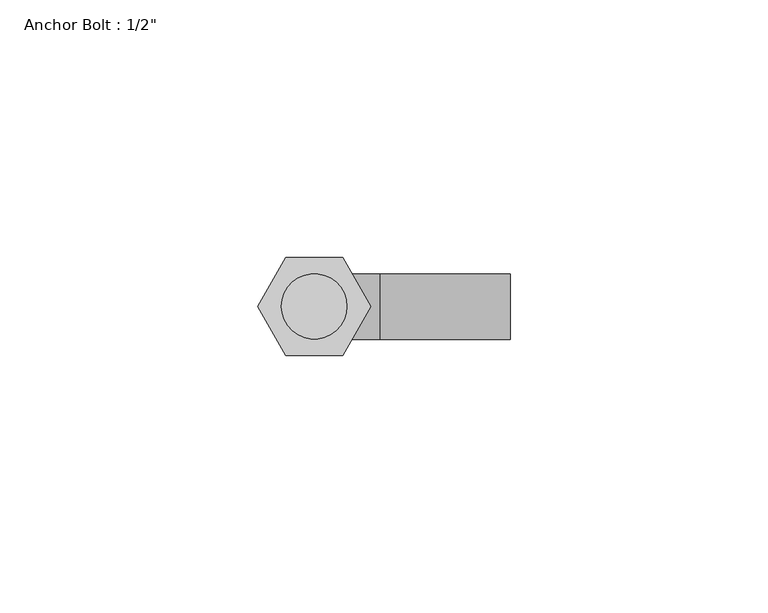
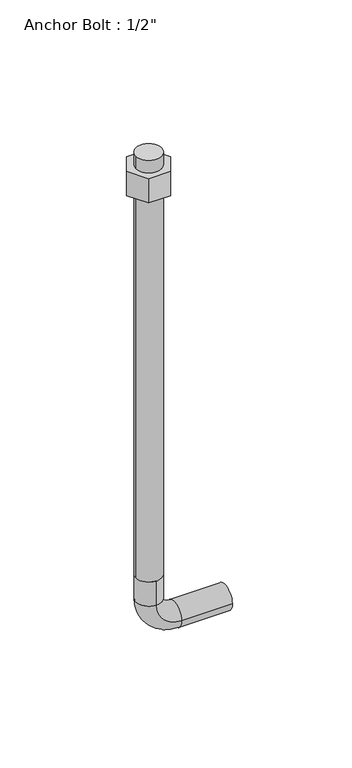
"""IFC4 building model written with IfcOpenShell, lengths in millimetres: fastener geometry."""

import ifcopenshell
import ifcopenshell.guid

model = None  # the IFC model being written
_history = None  # IfcOwnerHistory: only IFC2X3 demands one
_inside = {}  # id of a spatial element -> (the spatial element, [elements in it])
_under = {}  # id of a project, library or spatial element -> (it, [spatial elements below it])
_declared = {}  # id of a project -> (the project, [libraries it declares])
_typed = {}  # id of a type object -> (the type object, [elements of that type])
_made_of = {}  # id of a material, layer set ... -> (it, [elements and type objects made of it])


def new_model(schema):
    """Start an empty IFC model of exactly this schema.

    Asked for "IFC4X3", IfcOpenShell would pick the latest addendum, in which some entities
    have other attributes; the version numbers below select the first issue.
    IFC2X3 requires an IfcOwnerHistory on every rooted entity: one is made here for all.
    """
    global model, _history
    if schema == "IFC4X3":
        model = ifcopenshell.file(schema_version=(4, 3, 0, 0))
    else:
        model = ifcopenshell.file(schema=schema)
    _inside.clear()
    _under.clear()
    _declared.clear()
    _typed.clear()
    _made_of.clear()
    _history = None
    if model.schema == "IFC2X3":
        org = make("IfcOrganization", Name="unknown")
        user = make(
            "IfcPersonAndOrganization",
            ThePerson=make("IfcPerson", FamilyName="unknown"),
            TheOrganization=org,
        )
        app = make(
            "IfcApplication",
            ApplicationDeveloper=org,
            Version="unknown",
            ApplicationFullName="unknown",
            ApplicationIdentifier="unknown",
        )
        _history = make(
            "IfcOwnerHistory",
            OwningUser=user,
            OwningApplication=app,
            ChangeAction="ADDED",
            CreationDate=0,
        )
    return model


def make(cls, **values):
    """One entity of the class cls with the attributes given. An attribute that is None is left unset."""
    return model.create_entity(
        cls, **{name: value for name, value in values.items() if value is not None}
    )


def rooted(cls, **values):
    """An entity with a GlobalId (a new one), such as an element, a storey or a relation."""
    return make(cls, GlobalId=ifcopenshell.guid.new(), OwnerHistory=_history, **values)


def si_unit(unit_type, name, prefix=None):
    """IfcSIUnit, for example si_unit("LENGTHUNIT", "METRE", prefix="MILLI")."""
    return make("IfcSIUnit", UnitType=unit_type, Prefix=prefix, Name=name)


def assignment(units):
    """IfcUnitAssignment: the units of a project."""
    return None if units is None else make("IfcUnitAssignment", Units=units)


def point(xyz):
    """IfcCartesianPoint."""
    return None if xyz is None else make("IfcCartesianPoint", Coordinates=xyz)


def direction(xyz):
    """IfcDirection."""
    return None if xyz is None else make("IfcDirection", DirectionRatios=xyz)


def frame(location, z_axis=None, x_axis=None):
    """IfcAxis2Placement3D, a coordinate frame: its origin and axes. An axis left out is left unset."""
    return make(
        "IfcAxis2Placement3D",
        Location=point(location),
        Axis=direction(z_axis),
        RefDirection=direction(x_axis),
    )


def origin():
    """The frame at (0, 0, 0) with its axes left unset."""
    return frame((0.0, 0.0, 0.0))


def origin_with_axes():
    """The frame at (0, 0, 0) with the z axis (0, 0, 1) and the x axis (1, 0, 0) written out."""
    return frame((0.0, 0.0, 0.0), z_axis=(0.0, 0.0, 1.0), x_axis=(1.0, 0.0, 0.0))


def place(relative_to, where):
    """IfcLocalPlacement: puts the frame where relative to a parent placement (None: the world)."""
    return make(
        "IfcLocalPlacement", PlacementRelTo=relative_to, RelativePlacement=where
    )


def context(
    kind, dimensions, precision=None, world=None, true_north=None, identifier=None
):
    """IfcGeometricRepresentationContext, for example the 3D "Model" context."""
    return make(
        "IfcGeometricRepresentationContext",
        ContextIdentifier=identifier,
        ContextType=kind,
        CoordinateSpaceDimension=dimensions,
        Precision=precision,
        WorldCoordinateSystem=world,
        TrueNorth=true_north,
    )


def project(units=None, contexts=None):
    """IfcProject with its units and contexts."""
    return rooted(
        "IfcProject",
        Name="project",
        RepresentationContexts=contexts,
        UnitsInContext=assignment(units),
    )


def spatial(cls, under=None, at=None, **own):
    """A site, building, storey or space (cls), placed at a placement, below another one or the project."""
    s = rooted(cls, ObjectPlacement=at, **own)
    if under is not None:
        _under.setdefault(under.id(), (under, []))[1].append(s)
    return s


def polyline(points):
    """IfcPolyline through the points."""
    return make("IfcPolyline", Points=[point(p) for p in points])


def circle_curve(where, radius):
    """IfcCircle in the frame where."""
    return make("IfcCircle", Position=where, Radius=radius)


def ellipse_curve(where, semi_axis1, semi_axis2):
    """IfcEllipse in the frame where."""
    return make(
        "IfcEllipse", Position=where, SemiAxis1=semi_axis1, SemiAxis2=semi_axis2
    )


def trimmed(basis, trim1, trim2, sense, master):
    """IfcTrimmedCurve: the piece of a basis curve between two trims."""
    return make(
        "IfcTrimmedCurve",
        BasisCurve=basis,
        Trim1=trim1,
        Trim2=trim2,
        SenseAgreement=sense,
        MasterRepresentation=master,
    )


def outline(outer, holes=None, kind="AREA"):
    """IfcArbitraryClosedProfileDef: a profile drawn as a closed curve; with holes, ...WithVoids."""
    if holes is None:
        return make("IfcArbitraryClosedProfileDef", ProfileType=kind, OuterCurve=outer)
    return make(
        "IfcArbitraryProfileDefWithVoids",
        ProfileType=kind,
        OuterCurve=outer,
        InnerCurves=holes,
    )


def extrude(swept, where, along, depth):
    """IfcExtrudedAreaSolid: the profile swept, set in the frame where, extruded along a direction by depth."""
    return make(
        "IfcExtrudedAreaSolid",
        SweptArea=swept,
        Position=where,
        ExtrudedDirection=direction(along),
        Depth=depth,
    )


def shape(context_of_items, identifier, shape_type, items):
    """IfcShapeRepresentation: the items that make up one representation, for example the "Body"."""
    return make(
        "IfcShapeRepresentation",
        ContextOfItems=context_of_items,
        RepresentationIdentifier=identifier,
        RepresentationType=shape_type,
        Items=items,
    )


def source(mapping_origin, context_of_items, identifier, shape_type, items):
    """IfcRepresentationMap: a shape defined once, which mapped items show again and again."""
    return make(
        "IfcRepresentationMap",
        MappingOrigin=mapping_origin,
        MappedRepresentation=shape(context_of_items, identifier, shape_type, items),
    )


def transform(
    local_origin,
    x_axis=None,
    y_axis=None,
    z_axis=None,
    scale=None,
    scale2=None,
    scale3=None,
    uniform=True,
):
    """IfcCartesianTransformationOperator3D, or its non-uniform kind. x_axis, y_axis, z_axis: its Axis1, 2, 3."""
    if uniform:
        return make(
            "IfcCartesianTransformationOperator3D",
            Axis1=direction(x_axis),
            Axis2=direction(y_axis),
            LocalOrigin=point(local_origin),
            Scale=scale,
            Axis3=direction(z_axis),
        )
    return make(
        "IfcCartesianTransformationOperator3DnonUniform",
        Axis1=direction(x_axis),
        Axis2=direction(y_axis),
        LocalOrigin=point(local_origin),
        Scale=scale,
        Axis3=direction(z_axis),
        Scale2=scale2,
        Scale3=scale3,
    )


def mapped(mapping_source, mapping_target):
    """IfcMappedItem: shows the shape of a source again, moved by a transform."""
    return make(
        "IfcMappedItem", MappingSource=mapping_source, MappingTarget=mapping_target
    )


def made_of(thing, what):
    """Note that an element or type object is made of a material, layer set ...; save() writes the relation."""
    if what is not None:
        _made_of.setdefault(what.id(), (what, []))[1].append(thing)
    return thing


def element(
    cls,
    number,
    at=None,
    inside=None,
    cuts=None,
    type_object=None,
    material=None,
    context=None,
    identifier="Body",
    shape_type=None,
    held_by="IfcProductDefinitionShape",
    body=None,
    shapes=None,
    **own,
):
    """One element of the class cls, such as IfcWall. Its Tag is "e" and its number.

    at: its placement. inside: the storey or other place that contains it. cuts: it is an
    opening in that element (IfcRelVoidsElement). A single representation is given by context,
    identifier, shape_type and body (its items); several are given by shapes. held_by: the class
    of the entity that holds the representations. save() writes the other relations.
    """
    e = rooted(cls, Tag="e%d" % number, ObjectPlacement=at, **own)
    if body is not None:
        shapes = [shape(context, identifier, shape_type, body)]
    if shapes is not None:
        e.Representation = make(held_by, Representations=shapes)
    if inside is not None:
        _inside.setdefault(inside.id(), (inside, []))[1].append(e)
    if cuts is not None:
        rooted(
            "IfcRelVoidsElement", RelatingBuildingElement=cuts, RelatedOpeningElement=e
        )
    if type_object is not None:
        _typed.setdefault(type_object.id(), (type_object, []))[1].append(e)
    return made_of(e, material)


def aggregate(whole, parts):
    """IfcRelAggregates: a whole, such as a stair, and the parts it consists of."""
    return rooted("IfcRelAggregates", RelatingObject=whole, RelatedObjects=parts)


def save(model, path):
    """Write the relations noted so far, then the file.

    IfcRelAggregates (storeys below a building ...), IfcRelContainedInSpatialStructure (elements
    in a storey), IfcRelDefinesByType, IfcRelAssociatesMaterial and IfcRelDeclares: one each for
    every whole, place, type object, material and project.
    """
    for whole, parts in _under.values():
        aggregate(whole, parts)
    for where, things in _inside.values():
        rooted(
            "IfcRelContainedInSpatialStructure",
            RelatedElements=things,
            RelatingStructure=where,
        )
    for kind, things in _typed.values():
        rooted("IfcRelDefinesByType", RelatedObjects=things, RelatingType=kind)
    for what, things in _made_of.values():
        rooted("IfcRelAssociatesMaterial", RelatedObjects=things, RelatingMaterial=what)
    for by, libraries in _declared.values():
        rooted("IfcRelDeclares", RelatingContext=by, RelatedDefinitions=libraries)
    model.write(path)


def plane_surface(at):
    """IfcPlane: the flat surface through the origin of the frame at, square to its z axis."""
    return make("IfcPlane", Position=at)


def cylinder_surface(at, radius):
    """IfcCylindricalSurface: all points at the distance radius from the z axis of the frame at."""
    return make("IfcCylindricalSurface", Position=at, Radius=radius)


def revolved_surface(curve, axis_point, axis_direction):
    """IfcSurfaceOfRevolution: the curve turned about the line through axis_point along axis_direction."""
    return make(
        "IfcSurfaceOfRevolution",
        SweptCurve=make("IfcArbitraryOpenProfileDef", ProfileType="CURVE", Curve=curve),
        AxisPosition=make("IfcAxis1Placement", Location=point(axis_point), Axis=direction(axis_direction)),
    )


def advanced_brep(points, edges, surfaces, faces):
    """IfcAdvancedBrep: a solid bounded by faces that lie on surfaces and meet in shared edges.

    An edge is (start, end): straight between two places in points (the first is 0);
    or (start, end, curve); or (start, end, curve, False) where it runs against its curve.
    A face is (place in surfaces, loops), or (place, loops, False) where it looks against
    its surface's normal. A loop lists edges by number (the first is 1), with a minus sign
    where the edge is run from its end to its start. The first loop is the outer one.
    """
    corners = [point(p) for p in points]
    vertices = [make("IfcVertexPoint", VertexGeometry=c) for c in corners]
    made = []
    for start, end, *more in edges:
        made.append(
            make(
                "IfcEdgeCurve",
                EdgeStart=vertices[start],
                EdgeEnd=vertices[end],
                EdgeGeometry=more[0] if more else make("IfcPolyline", Points=[corners[start], corners[end]]),
                SameSense=more[1] if len(more) > 1 else True,
            )
        )
    hull = []
    for where, loops, *sense in faces:
        bounds = []
        for j, loop in enumerate(loops):
            ring = [make("IfcOrientedEdge", EdgeElement=made[abs(k) - 1], Orientation=k > 0) for k in loop]
            bounds.append(
                make(
                    "IfcFaceOuterBound" if j == 0 else "IfcFaceBound",
                    Bound=make("IfcEdgeLoop", EdgeList=ring),
                    Orientation=True,
                )
            )
        hull.append(make("IfcAdvancedFace", Bounds=bounds, FaceSurface=surfaces[where], SameSense=sense[0] if sense else True))
    return make("IfcAdvancedBrep", Outer=make("IfcClosedShell", CfsFaces=hull))


def fastener_5f8ddbac(model_context):
    return source(origin(), model_context, "Body", "SolidModel", [
        advanced_brep(
        [(-6.35, 0.0, 19.05), (6.35, 0.0, 19.05), (-6.35, 0.0, -203.2), (0.0, -6.35, -203.2), (6.35, 0.0, -203.2), (0.0, 6.35, -203.2), (0.0, 6.35, -215.9), (0.0, -6.35, -215.9), (12.7, 6.35, -228.6), (12.7, -6.35, -228.6), (38.1, 6.35, -228.6), (38.1, -6.35, -228.6)],
        [
            (0, 1, circle_curve(frame((0.0, 0.0, 19.05), z_axis=(0.0, 0.0, 1.0), x_axis=(1.0, 0.0, 0.0)), 6.35)),
            (1, 0, circle_curve(frame((0.0, 0.0, 19.05), z_axis=(0.0, 0.0, 1.0), x_axis=(1.0, 0.0, 0.0)), 6.35)),
            (0, 2),
            (2, 3, circle_curve(frame((0.0, 0.0, -203.2), z_axis=(0.0, 0.0, 1.0), x_axis=(1.0, 0.0, 0.0)), 6.35)),
            (3, 4, circle_curve(frame((0.0, 0.0, -203.2), z_axis=(0.0, 0.0, 1.0), x_axis=(1.0, 0.0, 0.0)), 6.35)),
            (4, 1),
            (4, 5, circle_curve(frame((0.0, 0.0, -203.2), z_axis=(0.0, 0.0, 1.0), x_axis=(1.0, 0.0, 0.0)), 6.35)),
            (5, 2, circle_curve(frame((0.0, 0.0, -203.2), z_axis=(0.0, 0.0, 1.0), x_axis=(1.0, 0.0, 0.0)), 6.35)),
            (5, 6),
            (6, 7, circle_curve(frame((0.0, 0.0, -215.9), z_axis=(0.0, 0.0, 1.0), x_axis=(0.0, -1.0, 0.0)), 6.35)),
            (7, 3),
            (7, 6, circle_curve(frame((0.0, 0.0, -215.9), z_axis=(0.0, 0.0, 1.0), x_axis=(0.0, -1.0, 0.0)), 6.35)),
            (6, 8, circle_curve(frame((12.7, 6.35, -215.9), z_axis=(0.0, -1.0, 0.0), x_axis=(-1.0, 0.0, 0.0)), 12.7)),
            (8, 9, circle_curve(frame((12.7, 0.0, -228.6), z_axis=(-1.0, 0.0, 0.0), x_axis=(0.0, -1.0, 0.0)), 6.35)),
            (9, 7, circle_curve(frame((12.7, -6.35, -215.9), z_axis=(0.0, 1.0, 0.0), x_axis=(-1.0, 0.0, 0.0)), 12.7)),
            (9, 8, circle_curve(frame((12.7, 0.0, -228.6), z_axis=(-1.0, 0.0, 0.0), x_axis=(0.0, -1.0, 0.0)), 6.35)),
            (10, 11, circle_curve(frame((38.1, 0.0, -228.6), z_axis=(1.0, 0.0, 0.0), x_axis=(0.0, -1.0, 0.0)), 6.35)),
            (11, 10, circle_curve(frame((38.1, 0.0, -228.6), z_axis=(1.0, 0.0, 0.0), x_axis=(0.0, -1.0, 0.0)), 6.35)),
            (8, 10),
            (11, 9),
        ],
        [
            plane_surface(frame((6.35, 0.0, 19.05), z_axis=(0.0, 0.0, 1.0), x_axis=(0.0, 1.0, 0.0))),
            cylinder_surface(frame((0.0, 0.0, -203.2), z_axis=(0.0, 0.0, 1.0), x_axis=(1.0, 0.0, 0.0)), 6.35),
            cylinder_surface(frame((0.0, 0.0, -203.2), z_axis=(0.0, 0.0, 1.0), x_axis=(0.0, -1.0, 0.0)), 6.35),
            revolved_surface(trimmed(ellipse_curve(frame((0.0, 0.0, -215.9), z_axis=(0.0, 0.0, 1.0), x_axis=(0.0, -1.0, 0.0)), 6.35, 6.35), [point((0.0, 6.35, -215.9))], [point((0.0, -6.35, -215.9))], True, "CARTESIAN"), (12.7, 0.0, -215.9), (0.0, -1.0, 0.0)),
            revolved_surface(trimmed(ellipse_curve(frame((0.0, 0.0, -215.9), z_axis=(0.0, 0.0, 1.0), x_axis=(0.0, -1.0, 0.0)), 6.35, 6.35), [point((0.0, -6.35, -215.9))], [point((0.0, 6.35, -215.9))], True, "CARTESIAN"), (12.7, 0.0, -215.9), (0.0, -1.0, 0.0)),
            plane_surface(frame((38.1, 0.0, -228.6), z_axis=(1.0, 0.0, 0.0), x_axis=(0.0, -1.0, 0.0))),
            cylinder_surface(frame((12.7, 0.0, -228.6), z_axis=(-1.0, 0.0, 0.0), x_axis=(0.0, -1.0, 0.0)), 6.35),
        ],
        [
            (0, [[1, 2]]),
            (1, [[-1, 3, 4, 5, 6]]),
            (1, [[-2, -6, 7, 8, -3]]),
            (2, [[9, 10, 11, -4, -8]]),
            (2, [[-9, -7, -5, -11, 12]]),
            (3, [[-10, 13, 14, 15]]),
            (4, [[-12, -15, 16, -13]]),
            (5, [[17, 18]]),
            (6, [[-14, 19, -18, 20]]),
            (6, [[-16, -20, -17, -19]]),
        ],
    ),
        extrude(outline(polyline([(-10.9985226, 0.0), (-5.4992613, 9.525), (5.4992613, 9.525), (10.9985226, 0.0), (5.4992613, -9.525), (-5.4992613, -9.525), (-10.9985226, 0.0)])), origin_with_axes(), (0.0, 0.0, 1.0), 12.7),
    ])


if __name__ == "__main__":
    model = new_model("IFC4")
    model_context = context("Model", 3, world=origin())
    ifc_project = project(units=[si_unit("LENGTHUNIT", "METRE", prefix="MILLI")], contexts=[model_context])
    site = spatial("IfcSite", under=ifc_project)
    building = spatial("IfcBuilding", under=site)
    placement = place(None, origin())
    fastener_shape = fastener_5f8ddbac(model_context)
    element("IfcFastener", 1, ObjectType="Anchor Bolt : 1/2\"", at=placement, inside=building, context=model_context, shape_type="MappedRepresentation", body=[
        mapped(fastener_shape, transform((0.0, 0.0, 0.0), x_axis=(1.0, 0.0, 0.0), y_axis=(0.0, 1.0, 0.0), z_axis=(0.0, 0.0, 1.0))),
    ])
    save(model, "model.ifc")

# Revit data of these elements
# Type "Anchor Bolt : 1/2\""
#   Side = 0' - 0 111/256"
#   Radius = 0' - 0 1/4"
#   Length = 0' - 8"
#   Head Size = 0' - 0 3/4"
#   Head Radius = 0' - 0 3/8"
#   Head Height = 0' - 0 1/2"
#   Diameter = 0' - 0 1/2"
#   Default Elevation = 4' - 0"
#   Bolt Material (Size) = 1/2" ANCHOR BOLTS (7" MIN. EMBED) AT 72" MIN O.C. SPACING (18" MAX. FROM CORNERS)
# Element 1 (IfcFastener, "Anchor Bolt : 1/2\"")
#   Materials on its faces: "1/2\" ANCHOR BOLTS (7\" MIN. EMBED) AT 72\" MIN O.C. SPACING (18\" MAX. FROM CORNERS)"
# Materials
#   "1/2\" ANCHOR BOLTS (7\" MIN. EMBED) AT 72\" MIN O.C. SPACING (18\" MAX. FROM CORNERS)": class "Generic", colour RGB 120 120 120, transparency 0, Cost = 0
